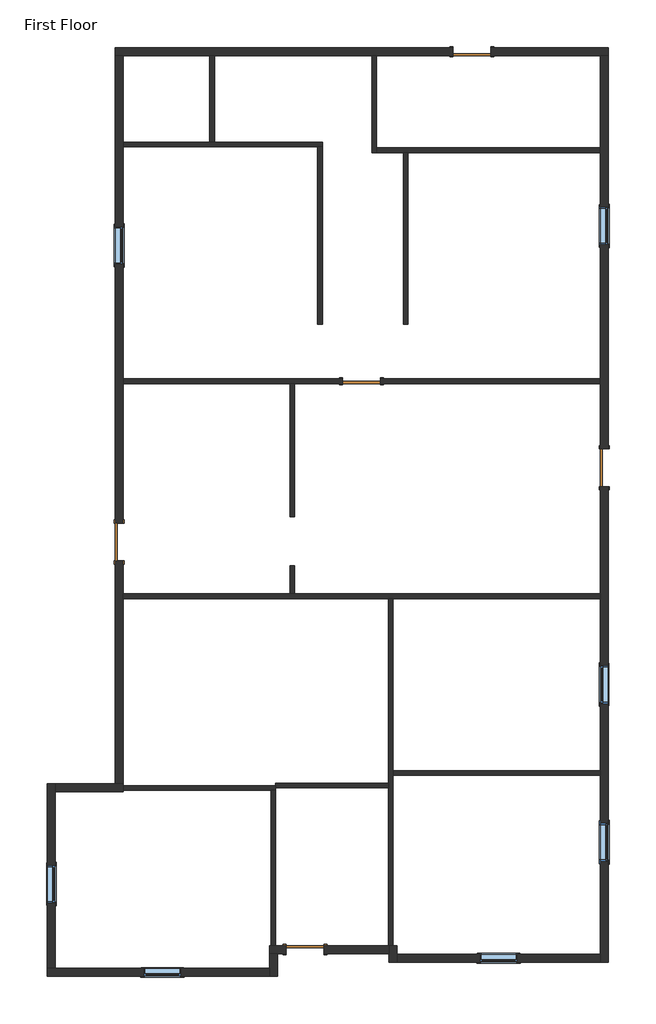
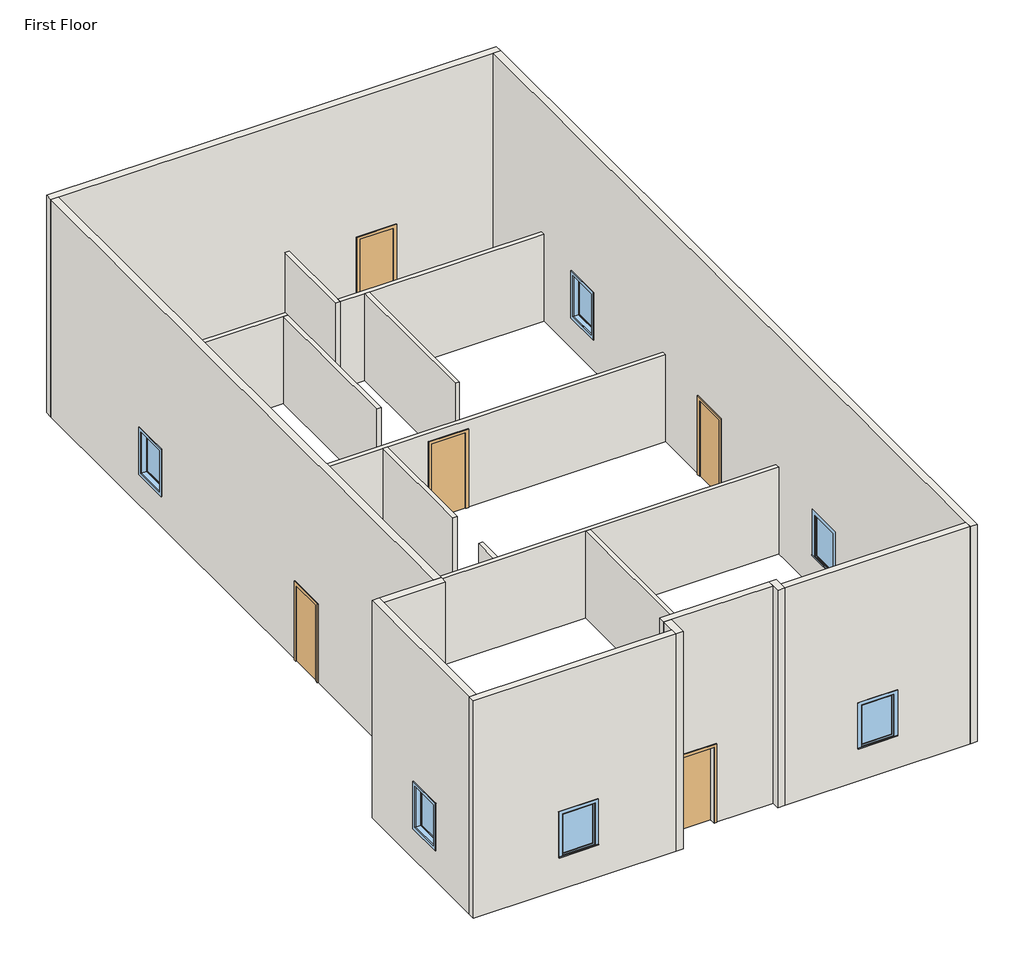
# One storey: 25 walls, 7 windows, 5 doors.
"""IFC4 building model written with IfcOpenShell, lengths in millimetres."""

import ifcopenshell
import ifcopenshell.guid

model = None  # the IFC model being written
_history = None  # IfcOwnerHistory: only IFC2X3 demands one
_inside = {}  # id of a spatial element -> (the spatial element, [elements in it])
_under = {}  # id of a project, library or spatial element -> (it, [spatial elements below it])
_declared = {}  # id of a project -> (the project, [libraries it declares])
_typed = {}  # id of a type object -> (the type object, [elements of that type])
_made_of = {}  # id of a material, layer set ... -> (it, [elements and type objects made of it])


def new_model(schema):
    """Start an empty IFC model of exactly this schema.

    Asked for "IFC4X3", IfcOpenShell would pick the latest addendum, in which some entities
    have other attributes; the version numbers below select the first issue.
    IFC2X3 requires an IfcOwnerHistory on every rooted entity: one is made here for all.
    """
    global model, _history
    if schema == "IFC4X3":
        model = ifcopenshell.file(schema_version=(4, 3, 0, 0))
    else:
        model = ifcopenshell.file(schema=schema)
    _inside.clear()
    _under.clear()
    _declared.clear()
    _typed.clear()
    _made_of.clear()
    _history = None
    if model.schema == "IFC2X3":
        org = make("IfcOrganization", Name="unknown")
        user = make(
            "IfcPersonAndOrganization",
            ThePerson=make("IfcPerson", FamilyName="unknown"),
            TheOrganization=org,
        )
        app = make(
            "IfcApplication",
            ApplicationDeveloper=org,
            Version="unknown",
            ApplicationFullName="unknown",
            ApplicationIdentifier="unknown",
        )
        _history = make(
            "IfcOwnerHistory",
            OwningUser=user,
            OwningApplication=app,
            ChangeAction="ADDED",
            CreationDate=0,
        )
    return model


def make(cls, **values):
    """One entity of the class cls with the attributes given. An attribute that is None is left unset."""
    return model.create_entity(
        cls, **{name: value for name, value in values.items() if value is not None}
    )


def rooted(cls, **values):
    """An entity with a GlobalId (a new one), such as an element, a storey or a relation."""
    return make(cls, GlobalId=ifcopenshell.guid.new(), OwnerHistory=_history, **values)


def si_unit(unit_type, name, prefix=None):
    """IfcSIUnit, for example si_unit("LENGTHUNIT", "METRE", prefix="MILLI")."""
    return make("IfcSIUnit", UnitType=unit_type, Prefix=prefix, Name=name)


def assignment(units):
    """IfcUnitAssignment: the units of a project."""
    return None if units is None else make("IfcUnitAssignment", Units=units)


def point(xyz):
    """IfcCartesianPoint."""
    return None if xyz is None else make("IfcCartesianPoint", Coordinates=xyz)


def direction(xyz):
    """IfcDirection."""
    return None if xyz is None else make("IfcDirection", DirectionRatios=xyz)


def frame(location, z_axis=None, x_axis=None):
    """IfcAxis2Placement3D, a coordinate frame: its origin and axes. An axis left out is left unset."""
    return make(
        "IfcAxis2Placement3D",
        Location=point(location),
        Axis=direction(z_axis),
        RefDirection=direction(x_axis),
    )


def origin():
    """The frame at (0, 0, 0) with its axes left unset."""
    return frame((0.0, 0.0, 0.0))


def origin_with_axes():
    """The frame at (0, 0, 0) with the z axis (0, 0, 1) and the x axis (1, 0, 0) written out."""
    return frame((0.0, 0.0, 0.0), z_axis=(0.0, 0.0, 1.0), x_axis=(1.0, 0.0, 0.0))


def place(relative_to, where):
    """IfcLocalPlacement: puts the frame where relative to a parent placement (None: the world)."""
    return make(
        "IfcLocalPlacement", PlacementRelTo=relative_to, RelativePlacement=where
    )


def context(
    kind, dimensions, precision=None, world=None, true_north=None, identifier=None
):
    """IfcGeometricRepresentationContext, for example the 3D "Model" context."""
    return make(
        "IfcGeometricRepresentationContext",
        ContextIdentifier=identifier,
        ContextType=kind,
        CoordinateSpaceDimension=dimensions,
        Precision=precision,
        WorldCoordinateSystem=world,
        TrueNorth=true_north,
    )


def project(units=None, contexts=None):
    """IfcProject with its units and contexts."""
    return rooted(
        "IfcProject",
        Name="project",
        RepresentationContexts=contexts,
        UnitsInContext=assignment(units),
    )


def spatial(cls, under=None, at=None, **own):
    """A site, building, storey or space (cls), placed at a placement, below another one or the project."""
    s = rooted(cls, ObjectPlacement=at, **own)
    if under is not None:
        _under.setdefault(under.id(), (under, []))[1].append(s)
    return s


def polyline(points):
    """IfcPolyline through the points."""
    return make("IfcPolyline", Points=[point(p) for p in points])


def outline(outer, holes=None, kind="AREA"):
    """IfcArbitraryClosedProfileDef: a profile drawn as a closed curve; with holes, ...WithVoids."""
    if holes is None:
        return make("IfcArbitraryClosedProfileDef", ProfileType=kind, OuterCurve=outer)
    return make(
        "IfcArbitraryProfileDefWithVoids",
        ProfileType=kind,
        OuterCurve=outer,
        InnerCurves=holes,
    )


def extrude(swept, where, along, depth):
    """IfcExtrudedAreaSolid: the profile swept, set in the frame where, extruded along a direction by depth."""
    return make(
        "IfcExtrudedAreaSolid",
        SweptArea=swept,
        Position=where,
        ExtrudedDirection=direction(along),
        Depth=depth,
    )


def faces_of(points, faces, orient=None, outer=None):
    """IfcFace entities. A face is a list of loops; a loop is a list of indices into points, from 0.

    orient and outer hold one flag for each loop. By default every Orientation is true, the
    first loop of a face is its IfcFaceOuterBound and the others are IfcFaceBound.
    """
    made = []
    for i, loops in enumerate(faces):
        bounds = []
        for j, loop in enumerate(loops):
            is_outer = j == 0 if outer is None else outer[i][j]
            bounds.append(
                make(
                    "IfcFaceOuterBound" if is_outer else "IfcFaceBound",
                    Bound=make("IfcPolyLoop", Polygon=[points[k] for k in loop]),
                    Orientation=True if orient is None else orient[i][j],
                )
            )
        made.append(make("IfcFace", Bounds=bounds))
    return made


def faceted_brep(points, faces, orient=None, outer=None, voids=None):
    """IfcFacetedBrep: a solid bounded by flat faces; with voids (closed shells), ...WithVoids."""
    shared = [point(p) for p in points]
    hull = make("IfcClosedShell", CfsFaces=faces_of(shared, faces, orient, outer))
    if voids is None:
        return make("IfcFacetedBrep", Outer=hull)
    return make(
        "IfcFacetedBrepWithVoids",
        Outer=hull,
        Voids=[
            make(cls, CfsFaces=faces_of(shared, fs, o, b)) for cls, fs, o, b in voids
        ],
    )


def shape(context_of_items, identifier, shape_type, items):
    """IfcShapeRepresentation: the items that make up one representation, for example the "Body"."""
    return make(
        "IfcShapeRepresentation",
        ContextOfItems=context_of_items,
        RepresentationIdentifier=identifier,
        RepresentationType=shape_type,
        Items=items,
    )


def source(mapping_origin, context_of_items, identifier, shape_type, items):
    """IfcRepresentationMap: a shape defined once, which mapped items show again and again."""
    return make(
        "IfcRepresentationMap",
        MappingOrigin=mapping_origin,
        MappedRepresentation=shape(context_of_items, identifier, shape_type, items),
    )


def transform(
    local_origin,
    x_axis=None,
    y_axis=None,
    z_axis=None,
    scale=None,
    scale2=None,
    scale3=None,
    uniform=True,
):
    """IfcCartesianTransformationOperator3D, or its non-uniform kind. x_axis, y_axis, z_axis: its Axis1, 2, 3."""
    if uniform:
        return make(
            "IfcCartesianTransformationOperator3D",
            Axis1=direction(x_axis),
            Axis2=direction(y_axis),
            LocalOrigin=point(local_origin),
            Scale=scale,
            Axis3=direction(z_axis),
        )
    return make(
        "IfcCartesianTransformationOperator3DnonUniform",
        Axis1=direction(x_axis),
        Axis2=direction(y_axis),
        LocalOrigin=point(local_origin),
        Scale=scale,
        Axis3=direction(z_axis),
        Scale2=scale2,
        Scale3=scale3,
    )


def mapped(mapping_source, mapping_target):
    """IfcMappedItem: shows the shape of a source again, moved by a transform."""
    return make(
        "IfcMappedItem", MappingSource=mapping_source, MappingTarget=mapping_target
    )


def made_of(thing, what):
    """Note that an element or type object is made of a material, layer set ...; save() writes the relation."""
    if what is not None:
        _made_of.setdefault(what.id(), (what, []))[1].append(thing)
    return thing


def element(
    cls,
    number,
    at=None,
    inside=None,
    cuts=None,
    type_object=None,
    material=None,
    context=None,
    identifier="Body",
    shape_type=None,
    held_by="IfcProductDefinitionShape",
    body=None,
    shapes=None,
    **own,
):
    """One element of the class cls, such as IfcWall. Its Tag is "e" and its number.

    at: its placement. inside: the storey or other place that contains it. cuts: it is an
    opening in that element (IfcRelVoidsElement). A single representation is given by context,
    identifier, shape_type and body (its items); several are given by shapes. held_by: the class
    of the entity that holds the representations. save() writes the other relations.
    """
    e = rooted(cls, Tag="e%d" % number, ObjectPlacement=at, **own)
    if body is not None:
        shapes = [shape(context, identifier, shape_type, body)]
    if shapes is not None:
        e.Representation = make(held_by, Representations=shapes)
    if inside is not None:
        _inside.setdefault(inside.id(), (inside, []))[1].append(e)
    if cuts is not None:
        rooted(
            "IfcRelVoidsElement", RelatingBuildingElement=cuts, RelatedOpeningElement=e
        )
    if type_object is not None:
        _typed.setdefault(type_object.id(), (type_object, []))[1].append(e)
    return made_of(e, material)


def aggregate(whole, parts):
    """IfcRelAggregates: a whole, such as a stair, and the parts it consists of."""
    return rooted("IfcRelAggregates", RelatingObject=whole, RelatedObjects=parts)


def save(model, path):
    """Write the relations noted so far, then the file.

    IfcRelAggregates (storeys below a building ...), IfcRelContainedInSpatialStructure (elements
    in a storey), IfcRelDefinesByType, IfcRelAssociatesMaterial and IfcRelDeclares: one each for
    every whole, place, type object, material and project.
    """
    for whole, parts in _under.values():
        aggregate(whole, parts)
    for where, things in _inside.values():
        rooted(
            "IfcRelContainedInSpatialStructure",
            RelatedElements=things,
            RelatingStructure=where,
        )
    for kind, things in _typed.values():
        rooted("IfcRelDefinesByType", RelatedObjects=things, RelatingType=kind)
    for what, things in _made_of.values():
        rooted("IfcRelAssociatesMaterial", RelatedObjects=things, RelatingMaterial=what)
    for by, libraries in _declared.values():
        rooted("IfcRelDeclares", RelatingContext=by, RelatedDefinitions=libraries)
    model.write(path)


def door_d6d25fb4(model_context):
    return source(origin(), model_context, "Body", "SweptSolid", [
        extrude(outline(polyline([(2209.8, -533.4), (0.0, -533.4), (0.0, -457.2), (2133.6, -457.2), (2133.6, 457.2), (0.0, 457.2), (0.0, 533.4), (2209.8, 533.4), (2209.8, -533.4)])), frame((0.0, 96.8375, 0.0), z_axis=(0.0, 1.0, 0.0), x_axis=(0.0, 0.0, 1.0)), (0.0, 0.0, 1.0), 25.4),
        extrude(outline(polyline([(2209.8, 533.4), (2209.8, -533.4), (0.0, -533.4), (0.0, -457.2), (2133.6, -457.2), (2133.6, 457.2), (0.0, 457.2), (0.0, 533.4), (2209.8, 533.4)])), frame((0.0, -122.2375, 0.0), z_axis=(0.0, 1.0, 0.0), x_axis=(0.0, 0.0, 1.0)), (0.0, 0.0, 1.0), 25.4),
        extrude(outline(polyline([(457.2, 46.0375), (-457.2, 46.0375), (-457.2, 96.8375), (457.2, 96.8375), (457.2, 46.0375)])), origin_with_axes(), (0.0, 0.0, 1.0), 2133.6),
    ])


def door_e5f9f3c4(model_context):
    return source(origin(), model_context, "Body", "SweptSolid", [
        extrude(outline(polyline([(2209.8, -533.4), (0.0, -533.4), (0.0, -457.2), (2133.6, -457.2), (2133.6, 457.2), (0.0, 457.2), (0.0, 533.4), (2209.8, 533.4), (2209.8, -533.4)])), frame((0.0, 57.15, 0.0), z_axis=(0.0, 1.0, 0.0), x_axis=(0.0, 0.0, 1.0)), (0.0, 0.0, 1.0), 25.4),
        extrude(outline(polyline([(2209.8, 533.4), (2209.8, -533.4), (0.0, -533.4), (0.0, -457.2), (2133.6, -457.2), (2133.6, 457.2), (0.0, 457.2), (0.0, 533.4), (2209.8, 533.4)])), frame((0.0, -82.55, 0.0), z_axis=(0.0, 1.0, 0.0), x_axis=(0.0, 0.0, 1.0)), (0.0, 0.0, 1.0), 25.4),
        extrude(outline(polyline([(457.2, 6.35), (-457.2, 6.35), (-457.2, 57.15), (457.2, 57.15), (457.2, 6.35)])), origin_with_axes(), (0.0, 0.0, 1.0), 2133.6),
    ])


def window_31be35ed(model_context):
    return source(origin(), model_context, "Body", "SweptSolid", [
        extrude(outline(polyline([(-565.15, 122.2375), (488.95, 122.2375), (488.95, 96.8375), (-565.15, 96.8375), (-565.15, 122.2375)])), frame((0.0, 0.0, 914.4), z_axis=(0.0, 0.0, 1.0), x_axis=(1.0, 0.0, 0.0)), (0.0, 0.0, 1.0), 19.05),
        extrude(outline(polyline([(2114.55, -476.25), (2114.55, 400.05), (933.45, 400.05), (933.45, 488.95), (2203.45, 488.95), (2203.45, -565.15), (933.45, -565.15), (933.45, -476.25), (2114.55, -476.25)])), frame((0.0, 96.8375, 0.0), z_axis=(0.0, 1.0, 0.0), x_axis=(0.0, 0.0, 1.0)), (0.0, 0.0, 1.0), 12.7),
        extrude(outline(polyline([(2190.75, 476.25), (2190.75, -552.45), (857.25, -552.45), (857.25, 476.25), (2190.75, 476.25)]), holes=[polyline([(2101.85, 387.35), (946.15, 387.35), (946.15, -463.55), (2101.85, -463.55), (2101.85, 387.35)])]), frame((0.0, -115.8875, 0.0), z_axis=(0.0, 1.0, 0.0), x_axis=(0.0, 0.0, 1.0)), (0.0, 0.0, 1.0), 19.05),
        extrude(outline(polyline([(355.6, 49.2125), (-431.8, 49.2125), (-431.8, 61.9125), (355.6, 61.9125), (355.6, 49.2125)])), frame((0.0, 0.0, 977.9), z_axis=(0.0, 0.0, 1.0), x_axis=(1.0, 0.0, 0.0)), (0.0, 0.0, 1.0), 1092.2),
        extrude(outline(polyline([(2114.55, -476.25), (933.45, -476.25), (933.45, 400.05), (2114.55, 400.05), (2114.55, -476.25)]), holes=[polyline([(2070.1, -431.8), (2070.1, 355.6), (977.9, 355.6), (977.9, -431.8), (2070.1, -431.8)])]), frame((0.0, 33.3375, 0.0), z_axis=(0.0, 1.0, 0.0), x_axis=(0.0, 0.0, 1.0)), (0.0, 0.0, 1.0), 44.45),
        extrude(outline(polyline([(2133.6, -495.3), (914.4, -495.3), (914.4, 419.1), (2133.6, 419.1), (2133.6, -495.3)]), holes=[polyline([(2101.85, -463.55), (2101.85, 387.35), (946.15, 387.35), (946.15, -463.55), (2101.85, -463.55)])]), frame((0.0, -96.8375, 0.0), z_axis=(0.0, 1.0, 0.0), x_axis=(0.0, 0.0, 1.0)), (0.0, 0.0, 1.0), 130.175),
        extrude(outline(polyline([(2133.6, 419.1), (2133.6, -495.3), (914.4, -495.3), (914.4, 419.1), (2133.6, 419.1)]), holes=[polyline([(2114.55, 400.05), (933.45, 400.05), (933.45, -476.25), (2114.55, -476.25), (2114.55, 400.05)])]), frame((0.0, 33.3375, 0.0), z_axis=(0.0, 1.0, 0.0), x_axis=(0.0, 0.0, 1.0)), (0.0, 0.0, 1.0), 63.5),
    ])


model = new_model("IFC4")

# Units and contexts
model_context = context("Model", 3, world=origin())
ifc_project = project(units=[si_unit("LENGTHUNIT", "METRE", prefix="MILLI")], contexts=[model_context])

# Site, building, storey
site = spatial("IfcSite", under=ifc_project)
building = spatial("IfcBuilding", under=site)
storey = spatial("IfcBuildingStorey", under=building, Name="First Floor", Elevation=0.0)

# Doors
placement = place(None, origin())
door_shape = door_d6d25fb4(model_context)
element("IfcDoor", 1, ObjectType="Single-Flush : 36\" x 84\"", at=placement, inside=storey, context=model_context, shape_type="MappedRepresentation", body=[
    mapped(door_shape, transform((2667.9934334, 17037.2838538, 0.0), x_axis=(0.0, 1.0, 0.0), y_axis=(-1.0, 0.0, 0.0), z_axis=(0.0, 0.0, 1.0))),
])
element("IfcDoor", 2, ObjectType="Single-Flush : 36\" x 84\"", at=placement, inside=storey, context=model_context, shape_type="MappedRepresentation", body=[
    mapped(door_shape, transform((14402.7934334, 18830.5238538, 0.0), x_axis=(0.0, 1.0, 0.0), y_axis=(-1.0, 0.0, 0.0), z_axis=(0.0, 0.0, 1.0))),
])
element("IfcDoor", 3, ObjectType="Single-Flush : 36\" x 84\"", at=placement, inside=storey, context=model_context, shape_type="MappedRepresentation", body=[
    mapped(door_shape, transform((7163.7934334, 7188.4338538, 0.0), x_axis=(1.0, 0.0, 0.0), y_axis=(0.0, 1.0, 0.0), z_axis=(0.0, 0.0, 1.0))),
])
element("IfcDoor", 4, ObjectType="Single-Flush : 36\" x 84\"", at=placement, inside=storey, context=model_context, shape_type="MappedRepresentation", body=[
    mapped(door_shape, transform((11202.3934334, 28888.9238538, 0.0), x_axis=(-1.0, 0.0, 0.0), y_axis=(0.0, -1.0, 0.0), z_axis=(0.0, 0.0, 1.0))),
])
door_2_shape = door_e5f9f3c4(model_context)
element("IfcDoor", 5, ObjectType="Single-Flush : 36\" x 84\"", at=placement, inside=storey, context=model_context, shape_type="MappedRepresentation", body=[
    mapped(door_2_shape, transform((8535.3934334, 20924.7538538, 0.0), x_axis=(-1.0, 0.0, 0.0), y_axis=(0.0, -1.0, 0.0), z_axis=(0.0, 0.0, 1.0))),
])

# Walls
element("IfcWall", 6, ObjectType="Generic - 8\" Masonry", at=placement, inside=storey, context=model_context, shape_type="Brep", body=[
    faceted_brep([(2571.1559334, 28792.0863538, 0.0), (2764.8309334, 28792.0863538, 0.0), (10745.1934334, 28792.0863538, 0.0), (10745.1934334, 28792.0863538, 2133.6), (11659.5934334, 28792.0863538, 2133.6), (11659.5934334, 28792.0863538, 0.0), (14305.9559334, 28792.0863538, 0.0), (14499.6309334, 28792.0863538, 0.0), (14499.6309334, 28792.0863538, 6096.0), (14305.9559334, 28792.0863538, 6096.0), (2764.8309334, 28792.0863538, 6096.0), (2571.1559334, 28792.0863538, 6096.0), (10745.1934334, 28985.7613538, 2133.6), (10745.1934334, 28985.7613538, 0.0), (2571.1559334, 28985.7613538, 0.0), (2571.1559334, 28985.7613538, 6096.0), (14499.6309334, 28985.7613538, 6096.0), (14499.6309334, 28985.7613538, 0.0), (11659.5934334, 28985.7613538, 0.0), (11659.5934334, 28985.7613538, 2133.6)], [[[0, 1, 2, 3, 4, 5, 6, 7, 8, 9, 10, 11]], [[12, 13, 14, 15, 16, 17, 18, 19]], [[18, 17, 7, 6, 5]], [[14, 13, 2, 1, 0]], [[11, 10, 9, 8, 16, 15]], [[8, 7, 17, 16]], [[0, 11, 15, 14]], [[3, 2, 13, 12]], [[4, 3, 12, 19]], [[5, 4, 19, 18]]]),
])
element("IfcWall", 7, ObjectType="Generic - 8\" Masonry", at=placement, inside=storey, context=model_context, shape_type="Brep", body=[
    faceted_brep([(14305.9559334, 28792.0863538, 0.0), (14305.9559334, 19287.7238538, 0.0), (14305.9559334, 19287.7238538, 2133.6), (14305.9559334, 18373.3238538, 2133.6), (14305.9559334, 18373.3238538, 0.0), (14305.9559334, 7075.7213538, 0.0), (14305.9559334, 6882.0463538, 0.0), (14305.9559334, 6882.0463538, 6096.0), (14305.9559334, 7075.7213538, 6096.0), (14305.9559334, 28792.0863538, 6096.0), (14305.9559334, 9323.3038538, 2133.6), (14305.9559334, 9323.3038538, 914.4), (14305.9559334, 10237.7038538, 914.4), (14305.9559334, 10237.7038538, 2133.6), (14305.9559334, 14048.3388538, 2133.6), (14305.9559334, 13133.9388538, 2133.6), (14305.9559334, 13133.9388538, 914.4), (14305.9559334, 14048.3388538, 914.4), (14305.9559334, 24220.0863538, 2133.6), (14305.9559334, 24220.0863538, 914.4), (14305.9559334, 25134.4863538, 914.4), (14305.9559334, 25134.4863538, 2133.6), (14499.6309334, 19287.7238538, 2133.6), (14499.6309334, 19287.7238538, 0.0), (14499.6309334, 28792.0863538, 0.0), (14499.6309334, 28792.0863538, 6096.0), (14499.6309334, 6882.0463538, 6096.0), (14499.6309334, 6882.0463538, 0.0), (14499.6309334, 18373.3238538, 0.0), (14499.6309334, 18373.3238538, 2133.6), (14499.6309334, 9323.3038538, 2133.6), (14499.6309334, 10237.7038538, 2133.6), (14499.6309334, 10237.7038538, 914.4), (14499.6309334, 9323.3038538, 914.4), (14499.6309334, 14048.3388538, 2133.6), (14499.6309334, 14048.3388538, 914.4), (14499.6309334, 13133.9388538, 914.4), (14499.6309334, 13133.9388538, 2133.6), (14499.6309334, 24220.0863538, 2133.6), (14499.6309334, 25134.4863538, 2133.6), (14499.6309334, 25134.4863538, 914.4), (14499.6309334, 24220.0863538, 914.4)], [[[0, 1, 2, 3, 4, 5, 6, 7, 8, 9], [10, 11, 12, 13], [14, 15, 16, 17], [18, 19, 20, 21]], [[22, 23, 24, 25, 26, 27, 28, 29], [30, 31, 32, 33], [34, 35, 36, 37], [38, 39, 40, 41]], [[28, 27, 6, 5, 4]], [[24, 23, 1, 0]], [[9, 8, 7, 26, 25]], [[0, 9, 25, 24]], [[7, 6, 27, 26]], [[2, 1, 23, 22]], [[3, 2, 22, 29]], [[4, 3, 29, 28]], [[11, 10, 30, 33]], [[12, 11, 33, 32]], [[13, 12, 32, 31]], [[10, 13, 31, 30]], [[35, 34, 14, 17]], [[36, 35, 17, 16]], [[37, 36, 16, 15]], [[34, 37, 15, 14]], [[19, 18, 38, 41]], [[20, 19, 41, 40]], [[21, 20, 40, 39]], [[18, 21, 39, 38]]]),
])
element("IfcWall", 8, ObjectType="Generic - 8\" Masonry", at=placement, inside=storey, context=model_context, shape_type="SweptSolid", body=[
    extrude(outline(polyline([(0.0, 14305.9559334), (6096.0, 14305.9559334), (6096.0, 9394.2309334), (0.0, 9394.2309334), (0.0, 14305.9559334)]), holes=[polyline([(2133.6, 11392.8934334), (2133.6, 12307.2934334), (914.4, 12307.2934334), (914.4, 11392.8934334), (2133.6, 11392.8934334)])]), frame((0.0, 6882.0463538, 0.0), z_axis=(0.0, 1.0, 0.0), x_axis=(0.0, 0.0, 1.0)), (0.0, 0.0, 1.0), 193.675),
])
element("IfcWall", 9, ObjectType="Generic - 8\" Masonry", at=placement, inside=storey, context=model_context, shape_type="Brep", body=[
    faceted_brep([(9394.2309334, 6882.0463538, 0.0), (9394.2309334, 7075.7213538, 0.0), (9394.2309334, 7285.2713538, 0.0), (9394.2309334, 7285.2713538, 6096.0), (9394.2309334, 7075.7213538, 6096.0), (9394.2309334, 6882.0463538, 6096.0), (9200.5559334, 6882.0463538, 0.0), (9200.5559334, 6882.0463538, 6096.0), (9200.5559334, 7091.5963538, 6096.0), (9200.5559334, 7285.2713538, 6096.0), (9200.5559334, 7285.2713538, 0.0), (9200.5559334, 7091.5963538, 0.0)], [[[0, 1, 2, 3, 4, 5]], [[6, 7, 8, 9, 10, 11]], [[2, 1, 0, 6, 11, 10]], [[5, 4, 3, 9, 8, 7]], [[0, 5, 7, 6]], [[2, 10, 9, 3]]]),
])
element("IfcWall", 10, ObjectType="Generic - 8\" Masonry", at=placement, inside=storey, context=model_context, shape_type="Brep", body=[
    faceted_brep([(9200.5559334, 7285.2713538, 0.0), (7620.9934334, 7285.2713538, 0.0), (7620.9934334, 7285.2713538, 2133.6), (6706.5934334, 7285.2713538, 2133.6), (6706.5934334, 7285.2713538, 0.0), (6304.9559334, 7285.2713538, 0.0), (6304.9559334, 7285.2713538, 6096.0), (9200.5559334, 7285.2713538, 6096.0), (7620.9934334, 7091.5963538, 2133.6), (7620.9934334, 7091.5963538, 0.0), (9200.5559334, 7091.5963538, 0.0), (9200.5559334, 7091.5963538, 6096.0), (6498.6309334, 7091.5963538, 6096.0), (6304.9559334, 7091.5963538, 6096.0), (6304.9559334, 7091.5963538, 0.0), (6498.6309334, 7091.5963538, 0.0), (6706.5934334, 7091.5963538, 0.0), (6706.5934334, 7091.5963538, 2133.6)], [[[0, 1, 2, 3, 4, 5, 6, 7]], [[8, 9, 10, 11, 12, 13, 14, 15, 16, 17]], [[10, 9, 1, 0]], [[16, 15, 14, 5, 4]], [[7, 6, 13, 12, 11]], [[2, 1, 9, 8]], [[3, 2, 8, 17]], [[4, 3, 17, 16]], [[5, 14, 13, 6]], [[7, 11, 10, 0]]]),
])
element("IfcWall", 11, ObjectType="Generic - 8\" Masonry", at=placement, inside=storey, context=model_context, shape_type="Brep", body=[
    faceted_brep([(6304.9559334, 7091.5963538, 6096.0), (6304.9559334, 7091.5963538, 0.0), (6304.9559334, 6732.8213538, 0.0), (6304.9559334, 6539.1463538, 0.0), (6304.9559334, 6539.1463538, 6096.0), (6304.9559334, 6732.8213538, 6096.0), (6498.6309334, 7091.5963538, 0.0), (6498.6309334, 7091.5963538, 6096.0), (6498.6309334, 6539.1463538, 6096.0), (6498.6309334, 6539.1463538, 0.0)], [[[0, 1, 2, 3, 4, 5]], [[6, 7, 8, 9]], [[3, 2, 1, 6, 9]], [[0, 5, 4, 8, 7]], [[4, 3, 9, 8]], [[0, 7, 6, 1]]]),
])
element("IfcWall", 12, ObjectType="Generic - 8\" Masonry", at=placement, inside=storey, context=model_context, shape_type="Brep", body=[
    faceted_brep([(6304.9559334, 6732.8213538, 0.0), (1126.5309334, 6732.8213538, 0.0), (932.8559334, 6732.8213538, 0.0), (932.8559334, 6732.8213538, 6096.0), (1126.5309334, 6732.8213538, 6096.0), (6304.9559334, 6732.8213538, 6096.0), (3258.5434334, 6732.8213538, 2133.6), (3258.5434334, 6732.8213538, 914.4), (4172.9434334, 6732.8213538, 914.4), (4172.9434334, 6732.8213538, 2133.6), (6304.9559334, 6539.1463538, 0.0), (6304.9559334, 6539.1463538, 6096.0), (932.8559334, 6539.1463538, 6096.0), (932.8559334, 6539.1463538, 0.0), (3258.5434334, 6539.1463538, 2133.6), (4172.9434334, 6539.1463538, 2133.6), (4172.9434334, 6539.1463538, 914.4), (3258.5434334, 6539.1463538, 914.4)], [[[0, 1, 2, 3, 4, 5], [6, 7, 8, 9]], [[10, 11, 12, 13], [14, 15, 16, 17]], [[2, 1, 0, 10, 13]], [[5, 4, 3, 12, 11]], [[0, 5, 11, 10]], [[3, 2, 13, 12]], [[7, 6, 14, 17]], [[8, 7, 17, 16]], [[9, 8, 16, 15]], [[6, 9, 15, 14]]]),
])
element("IfcWall", 13, ObjectType="Generic - 8\" Masonry", at=placement, inside=storey, context=model_context, shape_type="Brep", body=[
    faceted_brep([(1126.5309334, 6732.8213538, 0.0), (1126.5309334, 10996.8463538, 0.0), (1126.5309334, 11190.5213538, 0.0), (1126.5309334, 11190.5213538, 6096.0), (1126.5309334, 10996.8463538, 6096.0), (1126.5309334, 6732.8213538, 6096.0), (1126.5309334, 8312.3838538, 2133.6), (1126.5309334, 9226.7838538, 2133.6), (1126.5309334, 9226.7838538, 914.4), (1126.5309334, 8312.3838538, 914.4), (932.8559334, 6732.8213538, 0.0), (932.8559334, 6732.8213538, 6096.0), (932.8559334, 11190.5213538, 6096.0), (932.8559334, 11190.5213538, 0.0), (932.8559334, 8312.3838538, 2133.6), (932.8559334, 8312.3838538, 914.4), (932.8559334, 9226.7838538, 914.4), (932.8559334, 9226.7838538, 2133.6)], [[[0, 1, 2, 3, 4, 5], [6, 7, 8, 9]], [[10, 11, 12, 13], [14, 15, 16, 17]], [[2, 1, 0, 10, 13]], [[5, 4, 3, 12, 11]], [[0, 5, 11, 10]], [[3, 2, 13, 12]], [[15, 14, 6, 9]], [[16, 15, 9, 8]], [[17, 16, 8, 7]], [[14, 17, 7, 6]]]),
])
element("IfcWall", 14, ObjectType="Generic - 8\" Masonry", at=placement, inside=storey, context=model_context, shape_type="Brep", body=[
    faceted_brep([(1126.5309334, 10996.8463538, 0.0), (2764.8309334, 10996.8463538, 0.0), (2764.8309334, 10996.8463538, 6096.0), (1126.5309334, 10996.8463538, 6096.0), (1126.5309334, 11190.5213538, 0.0), (1126.5309334, 11190.5213538, 6096.0), (2571.1559334, 11190.5213538, 6096.0), (2764.8309334, 11190.5213538, 6096.0), (2764.8309334, 11190.5213538, 0.0), (2571.1559334, 11190.5213538, 0.0)], [[[0, 1, 2, 3]], [[4, 5, 6, 7, 8, 9]], [[1, 0, 4, 9, 8]], [[3, 2, 7, 6, 5]], [[0, 3, 5, 4]], [[1, 8, 7, 2]]]),
])
element("IfcWall", 15, ObjectType="Generic - 8\" Masonry", at=placement, inside=storey, context=model_context, shape_type="SweptSolid", body=[
    extrude(outline(polyline([(28792.0863538, 0.0), (17494.4838538, 0.0), (17494.4838538, 2133.6), (16580.0838538, 2133.6), (16580.0838538, 0.0), (11190.5213538, 0.0), (11190.5213538, 6096.0), (28792.0863538, 6096.0), (28792.0863538, 0.0)]), holes=[polyline([(23745.4238538, 2133.6), (23745.4238538, 914.4), (24659.8238538, 914.4), (24659.8238538, 2133.6), (23745.4238538, 2133.6)])]), frame((2571.1559334, 0.0, 0.0), z_axis=(1.0, 0.0, 0.0), x_axis=(0.0, 1.0, 0.0)), (0.0, 0.0, 1.0), 193.675),
])
element("IfcWall", 16, ObjectType="Interior - 4 1/2\" Partition", at=placement, inside=storey, context=model_context, shape_type="Brep", body=[
    faceted_brep([(2764.8309334, 26583.8738538, 0.0), (7468.5934334, 26583.8738538, 0.0), (7582.8934334, 26583.8738538, 0.0), (7582.8934334, 26583.8738538, 2438.4), (7468.5934334, 26583.8738538, 2438.4), (2764.8309334, 26583.8738538, 2438.4), (2764.8309334, 26698.1738538, 0.0), (2764.8309334, 26698.1738538, 2438.4), (4858.7434334, 26698.1738538, 2438.4), (4973.0434334, 26698.1738538, 2438.4), (7582.8934334, 26698.1738538, 2438.4), (7582.8934334, 26698.1738538, 0.0), (4973.0434334, 26698.1738538, 0.0), (4858.7434334, 26698.1738538, 0.0)], [[[0, 1, 2, 3, 4, 5]], [[6, 7, 8, 9, 10, 11, 12, 13]], [[2, 1, 0, 6, 13, 12, 11]], [[5, 4, 3, 10, 9, 8, 7]], [[0, 5, 7, 6]], [[3, 2, 11, 10]]]),
])
element("IfcWall", 17, ObjectType="Interior - 4 1/2\" Partition", at=placement, inside=storey, context=model_context, shape_type="SweptSolid", body=[
    extrude(outline(polyline([(4973.0434334, 28792.0863538), (4973.0434334, 26698.1738538), (4858.7434334, 26698.1738538), (4858.7434334, 28792.0863538), (4973.0434334, 28792.0863538)])), origin_with_axes(), (0.0, 0.0, 1.0), 2438.4),
])
element("IfcWall", 18, ObjectType="Interior - 4 1/2\" Partition", at=placement, inside=storey, context=model_context, shape_type="SweptSolid", body=[
    extrude(outline(polyline([(7468.5934334, 22297.6238538), (7468.5934334, 26583.8738538), (7582.8934334, 26583.8738538), (7582.8934334, 22297.6238538), (7468.5934334, 22297.6238538)])), origin_with_axes(), (0.0, 0.0, 1.0), 2438.4),
])
element("IfcWall", 19, ObjectType="Interior - 4 1/2\" Partition", at=placement, inside=storey, context=model_context, shape_type="Brep", body=[
    faceted_brep([(8783.0434334, 28792.0863538, 0.0), (8783.0434334, 26448.9363538, 0.0), (8783.0434334, 26448.9363538, 2438.4), (8783.0434334, 28792.0863538, 2438.4), (8897.3434334, 28792.0863538, 0.0), (8897.3434334, 28792.0863538, 2438.4), (8897.3434334, 26563.2363538, 2438.4), (8897.3434334, 26448.9363538, 2438.4), (8897.3434334, 26448.9363538, 0.0), (8897.3434334, 26563.2363538, 0.0)], [[[0, 1, 2, 3]], [[4, 5, 6, 7, 8, 9]], [[1, 0, 4, 9, 8]], [[3, 2, 7, 6, 5]], [[0, 3, 5, 4]], [[2, 1, 8, 7]]]),
])
element("IfcWall", 20, ObjectType="Interior - 4 1/2\" Partition", at=placement, inside=storey, context=model_context, shape_type="Brep", body=[
    faceted_brep([(8897.3434334, 26448.9363538, 0.0), (9545.0434334, 26448.9363538, 0.0), (9659.3434334, 26448.9363538, 0.0), (14305.9559334, 26448.9363538, 0.0), (14305.9559334, 26448.9363538, 2438.4), (9659.3434334, 26448.9363538, 2438.4), (9545.0434334, 26448.9363538, 2438.4), (8897.3434334, 26448.9363538, 2438.4), (8897.3434334, 26563.2363538, 0.0), (8897.3434334, 26563.2363538, 2438.4), (14305.9559334, 26563.2363538, 2438.4), (14305.9559334, 26563.2363538, 0.0)], [[[0, 1, 2, 3, 4, 5, 6, 7]], [[8, 9, 10, 11]], [[3, 2, 1, 0, 8, 11]], [[7, 6, 5, 4, 10, 9]], [[0, 7, 9, 8]], [[4, 3, 11, 10]]]),
])
element("IfcWall", 21, ObjectType="Interior - 4 1/2\" Partition", at=placement, inside=storey, context=model_context, shape_type="SweptSolid", body=[
    extrude(outline(polyline([(9545.0434334, 22297.6238538), (9545.0434334, 26448.9363538), (9659.3434334, 26448.9363538), (9659.3434334, 22297.6238538), (9545.0434334, 22297.6238538)])), origin_with_axes(), (0.0, 0.0, 1.0), 2438.4),
])
element("IfcWall", 22, ObjectType="Interior - 4 1/2\" Partition", at=placement, inside=storey, context=model_context, shape_type="Brep", body=[
    faceted_brep([(8078.1934334, 20981.9038538, 2133.6), (8078.1934334, 20981.9038538, 0.0), (2764.8309334, 20981.9038538, 0.0), (2764.8309334, 20981.9038538, 2438.4), (14305.9559334, 20981.9038538, 2438.4), (14305.9559334, 20981.9038538, 0.0), (8992.5934334, 20981.9038538, 0.0), (8992.5934334, 20981.9038538, 2133.6), (2764.8309334, 20867.6038538, 0.0), (6801.8434334, 20867.6038538, 0.0), (6916.1434334, 20867.6038538, 0.0), (8078.1934334, 20867.6038538, 0.0), (8078.1934334, 20867.6038538, 2133.6), (8992.5934334, 20867.6038538, 2133.6), (8992.5934334, 20867.6038538, 0.0), (14305.9559334, 20867.6038538, 0.0), (14305.9559334, 20867.6038538, 2438.4), (6916.1434334, 20867.6038538, 2438.4), (6801.8434334, 20867.6038538, 2438.4), (2764.8309334, 20867.6038538, 2438.4)], [[[0, 1, 2, 3, 4, 5, 6, 7]], [[8, 9, 10, 11, 12, 13, 14, 15, 16, 17, 18, 19]], [[6, 5, 15, 14]], [[2, 1, 11, 10, 9, 8]], [[4, 3, 19, 18, 17, 16]], [[5, 4, 16, 15]], [[3, 2, 8, 19]], [[12, 11, 1, 0]], [[13, 12, 0, 7]], [[14, 13, 7, 6]]]),
])
element("IfcWall", 23, ObjectType="Interior - 4 1/2\" Partition", at=placement, inside=storey, context=model_context, shape_type="SweptSolid", body=[
    extrude(outline(polyline([(6916.1434334, 20867.6038538), (6916.1434334, 17649.4238538), (6801.8434334, 17649.4238538), (6801.8434334, 20867.6038538), (6916.1434334, 20867.6038538)])), origin_with_axes(), (0.0, 0.0, 1.0), 2438.4),
])
element("IfcWall", 24, ObjectType="Interior - 4 1/2\" Partition", at=placement, inside=storey, context=model_context, shape_type="Brep", body=[
    faceted_brep([(2764.8309334, 15668.2238538, 0.0), (9183.0934334, 15668.2238538, 0.0), (9297.3934334, 15668.2238538, 0.0), (14305.9559334, 15668.2238538, 0.0), (14305.9559334, 15668.2238538, 2438.4), (9297.3934334, 15668.2238538, 2438.4), (9183.0934334, 15668.2238538, 2438.4), (2764.8309334, 15668.2238538, 2438.4), (2764.8309334, 15782.5238538, 0.0), (2764.8309334, 15782.5238538, 2438.4), (6801.8434334, 15782.5238538, 2438.4), (6916.1434334, 15782.5238538, 2438.4), (14305.9559334, 15782.5238538, 2438.4), (14305.9559334, 15782.5238538, 0.0), (6916.1434334, 15782.5238538, 0.0), (6801.8434334, 15782.5238538, 0.0)], [[[0, 1, 2, 3, 4, 5, 6, 7]], [[8, 9, 10, 11, 12, 13, 14, 15]], [[3, 2, 1, 0, 8, 15, 14, 13]], [[7, 6, 5, 4, 12, 11, 10, 9]], [[4, 3, 13, 12]], [[0, 7, 9, 8]]]),
])
element("IfcWall", 25, ObjectType="Interior - 4 1/2\" Partition", at=placement, inside=storey, context=model_context, shape_type="SweptSolid", body=[
    extrude(outline(polyline([(6801.8434334, 15782.5238538), (6801.8434334, 16468.3238538), (6916.1434334, 16468.3238538), (6916.1434334, 15782.5238538), (6801.8434334, 15782.5238538)])), origin_with_axes(), (0.0, 0.0, 1.0), 2438.4),
])
element("IfcWall", 26, ObjectType="Interior - 4 1/2\" Partition", at=placement, inside=storey, context=model_context, shape_type="Brep", body=[
    faceted_brep([(2764.8309334, 11036.5338538, 0.0), (6344.6434334, 11036.5338538, 0.0), (6458.9434334, 11036.5338538, 0.0), (6458.9434334, 11036.5338538, 2438.4), (6344.6434334, 11036.5338538, 2438.4), (2764.8309334, 11036.5338538, 2438.4), (2764.8309334, 11150.8338538, 0.0), (2764.8309334, 11150.8338538, 2438.4), (6458.9434334, 11150.8338538, 2438.4), (6458.9434334, 11150.8338538, 0.0), (6458.9434334, 11093.6838538, 0.0), (6458.9434334, 11093.6838538, 2438.4)], [[[0, 1, 2, 3, 4, 5]], [[6, 7, 8, 9]], [[2, 1, 0, 6, 9, 10]], [[5, 4, 3, 11, 8, 7]], [[0, 5, 7, 6]], [[3, 2, 10, 9, 8, 11]]]),
])
element("IfcWall", 27, ObjectType="Interior - 4 1/2\" Partition", at=placement, inside=storey, context=model_context, shape_type="SweptSolid", body=[
    extrude(outline(polyline([(6344.6434334, 7285.2713538), (6344.6434334, 11036.5338538), (6458.9434334, 11036.5338538), (6458.9434334, 7285.2713538), (6344.6434334, 7285.2713538)])), origin_with_axes(), (0.0, 0.0, 1.0), 2438.4),
])
element("IfcWall", 28, ObjectType="Interior - 4 1/2\" Partition", at=placement, inside=storey, context=model_context, shape_type="Brep", body=[
    faceted_brep([(9297.3934334, 7285.2713538, 0.0), (9297.3934334, 11399.7538538, 0.0), (9297.3934334, 11514.0538538, 0.0), (9297.3934334, 15668.2238538, 0.0), (9297.3934334, 15668.2238538, 2438.4), (9297.3934334, 11514.0538538, 2438.4), (9297.3934334, 11399.7538538, 2438.4), (9297.3934334, 7285.2713538, 2438.4), (9183.0934334, 7285.2713538, 0.0), (9183.0934334, 7285.2713538, 2438.4), (9183.0934334, 11093.6838538, 2438.4), (9183.0934334, 11207.9838538, 2438.4), (9183.0934334, 15668.2238538, 2438.4), (9183.0934334, 15668.2238538, 0.0), (9183.0934334, 11207.9838538, 0.0), (9183.0934334, 11093.6838538, 0.0)], [[[0, 1, 2, 3, 4, 5, 6, 7]], [[8, 9, 10, 11, 12, 13, 14, 15]], [[3, 2, 1, 0, 8, 15, 14, 13]], [[7, 6, 5, 4, 12, 11, 10, 9]], [[4, 3, 13, 12]], [[0, 7, 9, 8]]]),
])
element("IfcWall", 29, ObjectType="Interior - 4 1/2\" Partition", at=placement, inside=storey, context=model_context, shape_type="SweptSolid", body=[
    extrude(outline(polyline([(14305.9559334, 11399.7538538), (9297.3934334, 11399.7538538), (9297.3934334, 11514.0538538), (14305.9559334, 11514.0538538), (14305.9559334, 11399.7538538)])), origin_with_axes(), (0.0, 0.0, 1.0), 2438.4),
])
element("IfcWall", 30, ObjectType="Interior - 4 1/2\" Partition", at=placement, inside=storey, context=model_context, shape_type="Brep", body=[
    faceted_brep([(6458.9434334, 11093.6838538, 0.0), (9183.0934334, 11093.6838538, 0.0), (9183.0934334, 11093.6838538, 2438.4), (6458.9434334, 11093.6838538, 2438.4), (6458.9434334, 11207.9838538, 0.0), (6458.9434334, 11207.9838538, 2438.4), (9183.0934334, 11207.9838538, 2438.4), (9183.0934334, 11207.9838538, 0.0), (6458.9434334, 11150.8338538, 0.0), (6458.9434334, 11150.8338538, 2438.4)], [[[0, 1, 2, 3]], [[4, 5, 6, 7]], [[1, 0, 8, 4, 7]], [[3, 2, 6, 5, 9]], [[2, 1, 7, 6]], [[0, 3, 9, 5, 4, 8]]]),
])

# Windows
window_shape = window_31be35ed(model_context)
element("IfcWindow", 31, ObjectType="Fixed with Trim : 36\" x 48\"", at=placement, inside=storey, context=model_context, shape_type="MappedRepresentation", body=[
    mapped(window_shape, transform((11811.9934334, 6978.8838538, 0.0), x_axis=(-1.0, 0.0, 0.0), y_axis=(0.0, -1.0, 0.0), z_axis=(0.0, 0.0, 1.0))),
])
element("IfcWindow", 32, ObjectType="Fixed with Trim : 36\" x 48\"", at=placement, inside=storey, context=model_context, shape_type="MappedRepresentation", body=[
    mapped(window_shape, transform((3677.6434334, 6635.9838538, 0.0), x_axis=(-1.0, 0.0, 0.0), y_axis=(0.0, -1.0, 0.0), z_axis=(0.0, 0.0, 1.0))),
])
element("IfcWindow", 33, ObjectType="Fixed with Trim : 36\" x 48\"", at=placement, inside=storey, context=model_context, shape_type="MappedRepresentation", body=[
    mapped(window_shape, transform((1029.6934334, 8731.4838538, 0.0), x_axis=(0.0, -1.0, 0.0), y_axis=(1.0, 0.0, 0.0), z_axis=(0.0, 0.0, 1.0))),
])
element("IfcWindow", 34, ObjectType="Fixed with Trim : 36\" x 48\"", at=placement, inside=storey, context=model_context, shape_type="MappedRepresentation", body=[
    mapped(window_shape, transform((14402.7934334, 9742.4038538, 0.0), x_axis=(0.0, -1.0, 0.0), y_axis=(1.0, 0.0, 0.0), z_axis=(0.0, 0.0, 1.0))),
])
element("IfcWindow", 35, ObjectType="Fixed with Trim : 36\" x 48\"", at=placement, inside=storey, context=model_context, shape_type="MappedRepresentation", body=[
    mapped(window_shape, transform((14402.7934334, 13629.2388538, 0.0), x_axis=(0.0, 1.0, 0.0), y_axis=(-1.0, 0.0, 0.0), z_axis=(0.0, 0.0, 1.0))),
])
element("IfcWindow", 36, ObjectType="Fixed with Trim : 36\" x 48\"", at=placement, inside=storey, context=model_context, shape_type="MappedRepresentation", body=[
    mapped(window_shape, transform((14402.7934334, 24639.1863538, 0.0), x_axis=(0.0, -1.0, 0.0), y_axis=(1.0, 0.0, 0.0), z_axis=(0.0, 0.0, 1.0))),
])
element("IfcWindow", 37, ObjectType="Fixed with Trim : 36\" x 48\"", at=placement, inside=storey, context=model_context, shape_type="MappedRepresentation", body=[
    mapped(window_shape, transform((2667.9934334, 24164.5238538, 0.0), x_axis=(0.0, -1.0, 0.0), y_axis=(1.0, 0.0, 0.0), z_axis=(0.0, 0.0, 1.0))),
])

save(model, "model.ifc")

# Revit data of these elements
# Project information
#   Project Issue Date = "Issue Date"
#   Project Status = "Project Status"
#   Client Name = "Owner"
#   Project Address = "Enter address here"
#   Project Name = "Project Name"
#   Project Number = "Project Number"
# Type "Single-Flush : 36\" x 84\""
#   Type Mark = "34"
#   Assembly Code = "C1020"
#   Thickness = 0' - 2"
#   Height = 7' - 0"
#   Trim Projection Ext = 0' - 1"
#   Trim Projection Int = 0' - 1"
#   Trim Width = 0' - 3"
#   Width = 3' - 0"
#   Define Thermal Properties by = 0
#   Function = 0
#   Door Material = Door - Panel
#   Frame Material = Door - Frame
#   Wall Closure = (empty or 0)
# Type "Generic - 8\" Masonry"
#   Assembly Code = "B2010"
#   Layers, outside or top first: 0' - 7 5/8" "Concrete Masonry Units" (function 1)
# Type "Interior - 4 1/2\" Partition"
#   Assembly Code = "C1010145"
#   Layers, outside or top first: 0' - 0 1/2" "Gypsum Wall Board" (function 5); 0' - 3 1/2" "Softwood, Lumber" (function 1); 0' - 0 1/2" "Gypsum Wall Board" (function 5)
# Type "Fixed with Trim : 36\" x 48\""
#   Type Mark = "46"
#   Assembly Code = "B2020100"
#   Height = 4' - 0"
#   Default Sill Height = 3' - 0"
#   Trim Projection - Ext. = 0' - 0 1/2"
#   Trim Projection - Int. = 0' - 0 3/4"
#   Trim Width - Exterior = 0' - 3 1/2"
#   Trim Width - Interior = 0' - 3 1/2"
#   Width = 3' - 0"
#   Window Inset = 0' - 0 3/4"
#   Define Thermal Properties by = 0
#   Glass Pane Material = Glass
#   Sash Material = Sash
#   Trim Exterior Material = Trim
#   Trim Interior Material = Trim
#   Wall Closure = (empty or 0)
# Elements 1, 2, 3, 4, 5 (IfcDoor, "Single-Flush : 36\" x 84\"")
#   Phase Created = New Construction
#   Materials on its faces: "Door - Frame", "Door - Panel"
# Elements 6, 7, 8, 9, 10, 11, 12, 13, 14, 15 (IfcWall, "Generic - 8\" Masonry")
#   Top Offset = 0' - 0"
#   Base Offset = 0' - 0"
#   Unconnected Height = 20' - 0"
#   wall height = 20' - 0"
#   Phase Created = New Construction
#   Base Constraint = First Floor
#   Materials on its faces: "Concrete Masonry Units"
# Elements 16, 19, 26 (IfcWall, "Interior - 4 1/2\" Partition")
#   Top Offset = 0' - 0"
#   Base Offset = 0' - 0"
#   Unconnected Height = 8' - 0"
#   wall height = 8' - 0"
#   Phase Created = New Construction
#   Base Constraint = First Floor
#   Materials on its faces: "Gypsum Wall Board", "Default Wall"
# Elements 17, 18, 20, 21, 22, 23, 24, 25, 27, 28, 29, 30 (IfcWall, "Interior - 4 1/2\" Partition")
#   Top Offset = 0' - 0"
#   Base Offset = 0' - 0"
#   Unconnected Height = 8' - 0"
#   wall height = 8' - 0"
#   Phase Created = New Construction
#   Base Constraint = First Floor
#   Materials on its faces: "Default Wall", "Gypsum Wall Board"
# Element 31 (IfcWindow, "Fixed with Trim : 36\" x 48\"")
#   Mark = "8"
#   Phase Created = New Construction
#   Materials on its faces: "Sash", "Trim", "Glass"
# Element 32 (IfcWindow, "Fixed with Trim : 36\" x 48\"")
#   Mark = "9"
#   Phase Created = New Construction
#   Materials on its faces: "Sash", "Trim", "Glass"
# Element 33 (IfcWindow, "Fixed with Trim : 36\" x 48\"")
#   Mark = "10"
#   Phase Created = New Construction
#   Materials on its faces: "Sash", "Trim", "Glass"
# Element 34 (IfcWindow, "Fixed with Trim : 36\" x 48\"")
#   Mark = "11"
#   Phase Created = New Construction
#   Materials on its faces: "Sash", "Trim", "Glass"
# Element 35 (IfcWindow, "Fixed with Trim : 36\" x 48\"")
#   Mark = "12"
#   Phase Created = New Construction
#   Materials on its faces: "Sash", "Trim", "Glass"
# Element 36 (IfcWindow, "Fixed with Trim : 36\" x 48\"")
#   Mark = "13"
#   Phase Created = New Construction
#   Materials on its faces: "Sash", "Trim", "Glass"
# Element 37 (IfcWindow, "Fixed with Trim : 36\" x 48\"")
#   Mark = "14"
#   Phase Created = New Construction
#   Materials on its faces: "Sash", "Trim", "Glass"
# Materials
#   "Door - Panel": class "Wood", colour RGB 227 170 128, transparency 0, Cost = 0
#   "Door - Frame": class "Miscellaneous", colour RGB 153 76 43, transparency 0, Cost = 0
#   "Concrete Masonry Units": class "Masonry", colour RGB 152 154 138, transparency 0, Description = "Concrete masonry units", Cost = 0
#   "Gypsum Wall Board": class "Generic", colour RGB 228 228 228, transparency 0, Description = "Gypsum Wall Board", Cost = 0
#   "Softwood, Lumber": class "Wood", colour RGB 234 198 147, transparency 0, Description = "Pinus Echinata", Cost = 0
#   "Glass": class "Glass", colour RGB 236 240 239, transparency 0.5, Description = "Soda Lime Glass", Cost = 0
#   "Sash": class "Wood", colour RGB 227 170 128, transparency 0, Cost = 0
#   "Trim": class "Wood", colour RGB 227 170 128, transparency 0, Cost = 0
#   "Default Wall": class "Miscellaneous", colour RGB 80 80 80, transparency 0, Cost = 0
